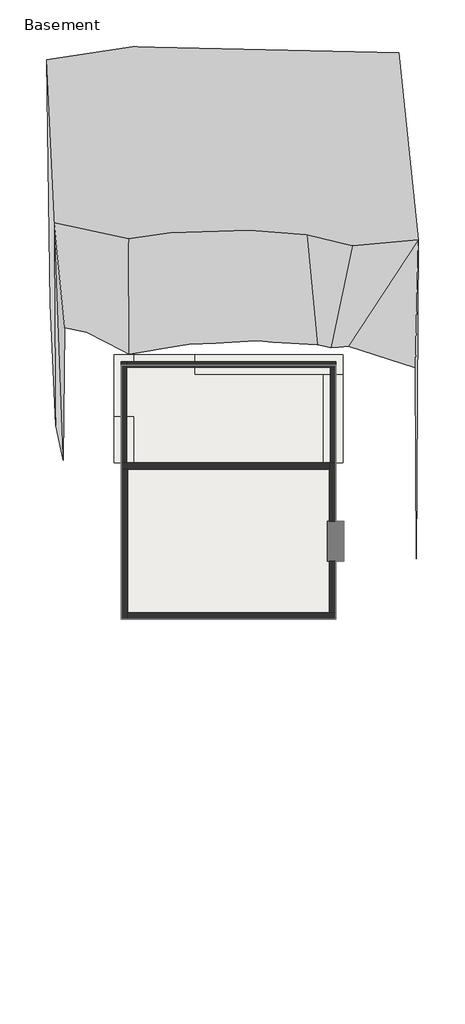
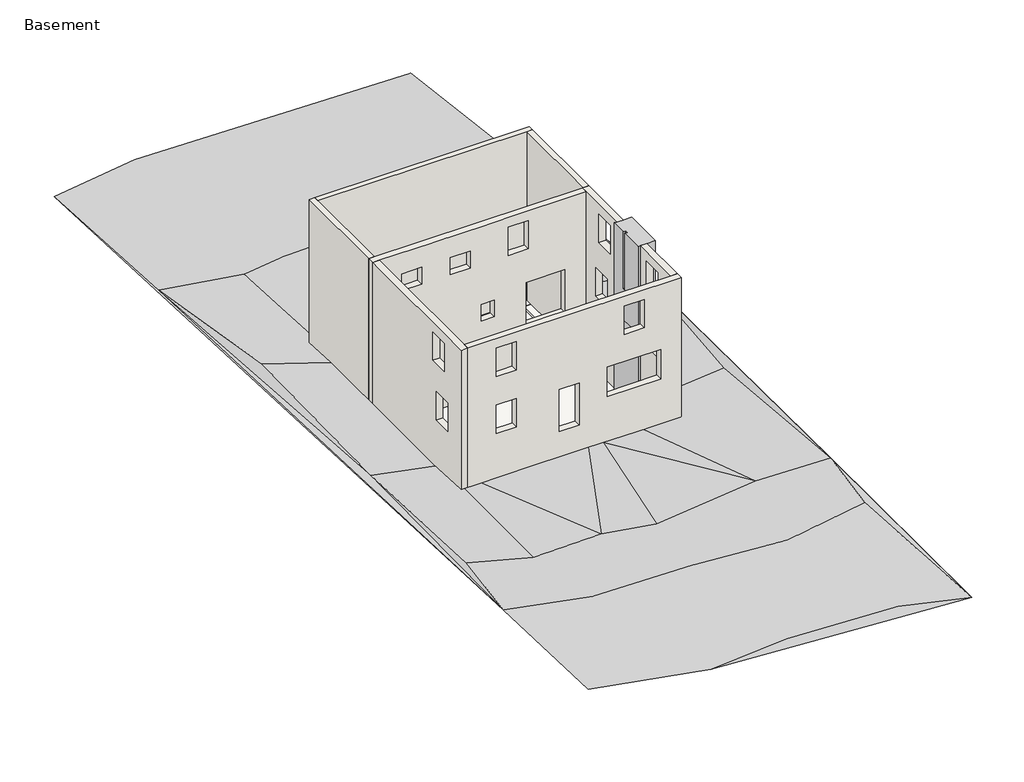
# One storey: 8 walls, 4 proxies, 3 footings, 2 slabs.
"""IFC4 building model written with IfcOpenShell, lengths in millimetres."""

import ifcopenshell
import ifcopenshell.guid

model = None  # the IFC model being written
_history = None  # IfcOwnerHistory: only IFC2X3 demands one
_inside = {}  # id of a spatial element -> (the spatial element, [elements in it])
_under = {}  # id of a project, library or spatial element -> (it, [spatial elements below it])
_declared = {}  # id of a project -> (the project, [libraries it declares])
_typed = {}  # id of a type object -> (the type object, [elements of that type])
_made_of = {}  # id of a material, layer set ... -> (it, [elements and type objects made of it])


def new_model(schema):
    """Start an empty IFC model of exactly this schema.

    Asked for "IFC4X3", IfcOpenShell would pick the latest addendum, in which some entities
    have other attributes; the version numbers below select the first issue.
    IFC2X3 requires an IfcOwnerHistory on every rooted entity: one is made here for all.
    """
    global model, _history
    if schema == "IFC4X3":
        model = ifcopenshell.file(schema_version=(4, 3, 0, 0))
    else:
        model = ifcopenshell.file(schema=schema)
    _inside.clear()
    _under.clear()
    _declared.clear()
    _typed.clear()
    _made_of.clear()
    _history = None
    if model.schema == "IFC2X3":
        org = make("IfcOrganization", Name="unknown")
        user = make(
            "IfcPersonAndOrganization",
            ThePerson=make("IfcPerson", FamilyName="unknown"),
            TheOrganization=org,
        )
        app = make(
            "IfcApplication",
            ApplicationDeveloper=org,
            Version="unknown",
            ApplicationFullName="unknown",
            ApplicationIdentifier="unknown",
        )
        _history = make(
            "IfcOwnerHistory",
            OwningUser=user,
            OwningApplication=app,
            ChangeAction="ADDED",
            CreationDate=0,
        )
    return model


def make(cls, **values):
    """One entity of the class cls with the attributes given. An attribute that is None is left unset."""
    return model.create_entity(
        cls, **{name: value for name, value in values.items() if value is not None}
    )


def rooted(cls, **values):
    """An entity with a GlobalId (a new one), such as an element, a storey or a relation."""
    return make(cls, GlobalId=ifcopenshell.guid.new(), OwnerHistory=_history, **values)


def si_unit(unit_type, name, prefix=None):
    """IfcSIUnit, for example si_unit("LENGTHUNIT", "METRE", prefix="MILLI")."""
    return make("IfcSIUnit", UnitType=unit_type, Prefix=prefix, Name=name)


def assignment(units):
    """IfcUnitAssignment: the units of a project."""
    return None if units is None else make("IfcUnitAssignment", Units=units)


def point(xyz):
    """IfcCartesianPoint."""
    return None if xyz is None else make("IfcCartesianPoint", Coordinates=xyz)


def direction(xyz):
    """IfcDirection."""
    return None if xyz is None else make("IfcDirection", DirectionRatios=xyz)


def frame(location, z_axis=None, x_axis=None):
    """IfcAxis2Placement3D, a coordinate frame: its origin and axes. An axis left out is left unset."""
    return make(
        "IfcAxis2Placement3D",
        Location=point(location),
        Axis=direction(z_axis),
        RefDirection=direction(x_axis),
    )


def origin():
    """The frame at (0, 0, 0) with its axes left unset."""
    return frame((0.0, 0.0, 0.0))


def place(relative_to, where):
    """IfcLocalPlacement: puts the frame where relative to a parent placement (None: the world)."""
    return make(
        "IfcLocalPlacement", PlacementRelTo=relative_to, RelativePlacement=where
    )


def context(
    kind, dimensions, precision=None, world=None, true_north=None, identifier=None
):
    """IfcGeometricRepresentationContext, for example the 3D "Model" context."""
    return make(
        "IfcGeometricRepresentationContext",
        ContextIdentifier=identifier,
        ContextType=kind,
        CoordinateSpaceDimension=dimensions,
        Precision=precision,
        WorldCoordinateSystem=world,
        TrueNorth=true_north,
    )


def project(units=None, contexts=None):
    """IfcProject with its units and contexts."""
    return rooted(
        "IfcProject",
        Name="project",
        RepresentationContexts=contexts,
        UnitsInContext=assignment(units),
    )


def spatial(cls, under=None, at=None, **own):
    """A site, building, storey or space (cls), placed at a placement, below another one or the project."""
    s = rooted(cls, ObjectPlacement=at, **own)
    if under is not None:
        _under.setdefault(under.id(), (under, []))[1].append(s)
    return s


def polyline(points):
    """IfcPolyline through the points."""
    return make("IfcPolyline", Points=[point(p) for p in points])


def point_list(points):
    """IfcCartesianPointList2D or 3D."""
    cls = (
        "IfcCartesianPointList2D" if len(points[0]) == 2 else "IfcCartesianPointList3D"
    )
    return make(cls, CoordList=points)


def outline(outer, holes=None, kind="AREA"):
    """IfcArbitraryClosedProfileDef: a profile drawn as a closed curve; with holes, ...WithVoids."""
    if holes is None:
        return make("IfcArbitraryClosedProfileDef", ProfileType=kind, OuterCurve=outer)
    return make(
        "IfcArbitraryProfileDefWithVoids",
        ProfileType=kind,
        OuterCurve=outer,
        InnerCurves=holes,
    )


def extrude(swept, where, along, depth):
    """IfcExtrudedAreaSolid: the profile swept, set in the frame where, extruded along a direction by depth."""
    return make(
        "IfcExtrudedAreaSolid",
        SweptArea=swept,
        Position=where,
        ExtrudedDirection=direction(along),
        Depth=depth,
    )


def faces_of(points, faces, orient=None, outer=None):
    """IfcFace entities. A face is a list of loops; a loop is a list of indices into points, from 0.

    orient and outer hold one flag for each loop. By default every Orientation is true, the
    first loop of a face is its IfcFaceOuterBound and the others are IfcFaceBound.
    """
    made = []
    for i, loops in enumerate(faces):
        bounds = []
        for j, loop in enumerate(loops):
            is_outer = j == 0 if outer is None else outer[i][j]
            bounds.append(
                make(
                    "IfcFaceOuterBound" if is_outer else "IfcFaceBound",
                    Bound=make("IfcPolyLoop", Polygon=[points[k] for k in loop]),
                    Orientation=True if orient is None else orient[i][j],
                )
            )
        made.append(make("IfcFace", Bounds=bounds))
    return made


def faceted_brep(points, faces, orient=None, outer=None, voids=None):
    """IfcFacetedBrep: a solid bounded by flat faces; with voids (closed shells), ...WithVoids."""
    shared = [point(p) for p in points]
    hull = make("IfcClosedShell", CfsFaces=faces_of(shared, faces, orient, outer))
    if voids is None:
        return make("IfcFacetedBrep", Outer=hull)
    return make(
        "IfcFacetedBrepWithVoids",
        Outer=hull,
        Voids=[
            make(cls, CfsFaces=faces_of(shared, fs, o, b)) for cls, fs, o, b in voids
        ],
    )


def triangles(points, corners, closed=None, point_numbers=None):
    """IfcTriangulatedFaceSet: each triangle names its three corners, points numbered from 1."""
    return make(
        "IfcTriangulatedFaceSet",
        Coordinates=point_list(points),
        Closed=closed,
        CoordIndex=corners,
        PnIndex=point_numbers,
    )


def shape(context_of_items, identifier, shape_type, items):
    """IfcShapeRepresentation: the items that make up one representation, for example the "Body"."""
    return make(
        "IfcShapeRepresentation",
        ContextOfItems=context_of_items,
        RepresentationIdentifier=identifier,
        RepresentationType=shape_type,
        Items=items,
    )


def source(mapping_origin, context_of_items, identifier, shape_type, items):
    """IfcRepresentationMap: a shape defined once, which mapped items show again and again."""
    return make(
        "IfcRepresentationMap",
        MappingOrigin=mapping_origin,
        MappedRepresentation=shape(context_of_items, identifier, shape_type, items),
    )


def transform(
    local_origin,
    x_axis=None,
    y_axis=None,
    z_axis=None,
    scale=None,
    scale2=None,
    scale3=None,
    uniform=True,
):
    """IfcCartesianTransformationOperator3D, or its non-uniform kind. x_axis, y_axis, z_axis: its Axis1, 2, 3."""
    if uniform:
        return make(
            "IfcCartesianTransformationOperator3D",
            Axis1=direction(x_axis),
            Axis2=direction(y_axis),
            LocalOrigin=point(local_origin),
            Scale=scale,
            Axis3=direction(z_axis),
        )
    return make(
        "IfcCartesianTransformationOperator3DnonUniform",
        Axis1=direction(x_axis),
        Axis2=direction(y_axis),
        LocalOrigin=point(local_origin),
        Scale=scale,
        Axis3=direction(z_axis),
        Scale2=scale2,
        Scale3=scale3,
    )


def mapped(mapping_source, mapping_target):
    """IfcMappedItem: shows the shape of a source again, moved by a transform."""
    return make(
        "IfcMappedItem", MappingSource=mapping_source, MappingTarget=mapping_target
    )


def made_of(thing, what):
    """Note that an element or type object is made of a material, layer set ...; save() writes the relation."""
    if what is not None:
        _made_of.setdefault(what.id(), (what, []))[1].append(thing)
    return thing


def element(
    cls,
    number,
    at=None,
    inside=None,
    cuts=None,
    type_object=None,
    material=None,
    context=None,
    identifier="Body",
    shape_type=None,
    held_by="IfcProductDefinitionShape",
    body=None,
    shapes=None,
    **own,
):
    """One element of the class cls, such as IfcWall. Its Tag is "e" and its number.

    at: its placement. inside: the storey or other place that contains it. cuts: it is an
    opening in that element (IfcRelVoidsElement). A single representation is given by context,
    identifier, shape_type and body (its items); several are given by shapes. held_by: the class
    of the entity that holds the representations. save() writes the other relations.
    """
    e = rooted(cls, Tag="e%d" % number, ObjectPlacement=at, **own)
    if body is not None:
        shapes = [shape(context, identifier, shape_type, body)]
    if shapes is not None:
        e.Representation = make(held_by, Representations=shapes)
    if inside is not None:
        _inside.setdefault(inside.id(), (inside, []))[1].append(e)
    if cuts is not None:
        rooted(
            "IfcRelVoidsElement", RelatingBuildingElement=cuts, RelatedOpeningElement=e
        )
    if type_object is not None:
        _typed.setdefault(type_object.id(), (type_object, []))[1].append(e)
    return made_of(e, material)


def aggregate(whole, parts):
    """IfcRelAggregates: a whole, such as a stair, and the parts it consists of."""
    return rooted("IfcRelAggregates", RelatingObject=whole, RelatedObjects=parts)


def save(model, path):
    """Write the relations noted so far, then the file.

    IfcRelAggregates (storeys below a building ...), IfcRelContainedInSpatialStructure (elements
    in a storey), IfcRelDefinesByType, IfcRelAssociatesMaterial and IfcRelDeclares: one each for
    every whole, place, type object, material and project.
    """
    for whole, parts in _under.values():
        aggregate(whole, parts)
    for where, things in _inside.values():
        rooted(
            "IfcRelContainedInSpatialStructure",
            RelatedElements=things,
            RelatingStructure=where,
        )
    for kind, things in _typed.values():
        rooted("IfcRelDefinesByType", RelatedObjects=things, RelatingType=kind)
    for what, things in _made_of.values():
        rooted("IfcRelAssociatesMaterial", RelatedObjects=things, RelatingMaterial=what)
    for by, libraries in _declared.values():
        rooted("IfcRelDeclares", RelatingContext=by, RelatedDefinitions=libraries)
    model.write(path)


def existing_fireplace_existing_fireplace_063a625f(model_context):
    return source(origin(), model_context, "Body", "Brep", [
        faceted_brep([(4450.2196932, 434.2888758, 5486.4), (4069.2196932, 434.2888758, 5486.4), (3764.4196932, 434.2888758, 5486.4), (3662.8196932, 434.2888758, 5486.4), (3662.8196932, -276.9111242, 5486.4), (3767.2567114, -276.9111242, 5486.4), (3767.2567114, -403.9111242, 5486.4), (3662.8196932, -403.9111242, 5486.4), (3662.8196932, -1445.3111242, 5486.4), (3764.4196932, -1445.3111242, 5486.4), (4069.2196932, -1445.3111242, 5486.4), (4450.2196932, -1445.3111242, 5486.4), (4450.2196932, 434.2888758, -2667.0), (4450.2196932, -1445.3111242, -2667.0), (4069.2196932, -1445.3111242, -2667.0), (3764.4196932, -1445.3111242, -2667.0), (3662.8196932, -1445.3111242, -2667.0), (3662.8196932, 434.2888758, -2667.0), (3764.4196932, 434.2888758, -2667.0), (4069.2196932, 434.2888758, -2667.0), (3662.8196932, -403.9111242, 2743.2), (3662.8196932, -276.9111242, 2743.2), (3662.8196932, 154.8888758, 0.0), (3662.8196932, 154.8888758, 1219.2), (3662.8196932, -1165.9111242, 1219.2), (3662.8196932, -1165.9111242, 0.0), (4145.4196932, -20.7631592, 1219.2), (4145.4196932, -990.2590891, 1219.2), (4145.4196932, -990.2590891, 0.0), (4145.4196932, -20.7631592, 0.0), (3767.2567114, -403.9111242, 2743.2), (3767.2567114, -276.9111242, 2743.2)], [[[0, 1, 2, 3, 4, 5, 6, 7, 8, 9, 10, 11]], [[12, 13, 14, 15, 16, 17, 18, 19]], [[3, 2, 1, 0, 12, 19, 18, 17]], [[3, 17, 16, 8, 7, 20, 21, 4], [22, 23, 24, 25]], [[11, 10, 9, 8, 16, 15, 14, 13]], [[0, 11, 13, 12]], [[24, 23, 26, 27]], [[25, 24, 27, 28]], [[27, 26, 29, 28]], [[23, 22, 29, 26]], [[22, 25, 28, 29]], [[6, 30, 20, 7]], [[31, 5, 4, 21]], [[30, 31, 21, 20]], [[30, 6, 5, 31]]]),
    ])


model = new_model("IFC4")

# Units and contexts
model_context = context("Model", 3, world=origin())
ifc_project = project(units=[si_unit("LENGTHUNIT", "METRE", prefix="MILLI")], contexts=[model_context])

# Site, building, storey
site = spatial("IfcSite", under=ifc_project)
building = spatial("IfcBuilding", under=site)
storey = spatial("IfcBuildingStorey", under=building, Name="Basement", Elevation=-2667.0)

# Proxies
placement = place(None, origin())
element("IfcBuildingElementProxy", 1, Name="Building Element Proxy", at=placement, inside=storey, context=model_context, shape_type="Tessellation", body=[
    triangles([(-9474.14729, 22003.2871765, -1727.1999516), (-8916.1412338, -12566.1132111, -939.7999758), (-8632.7724838, -18803.3999359, -1092.1999758), (-3754.3850807, -20036.8885986, -1092.1999758), (7677.2023224, -20906.8378235, -1092.1999758), (7936.7585724, 13587.9496765, -1752.6), (7012.0400162, 22339.8364014, -1727.1999516), (-5437.1349838, 22620.8239014, -1727.1999516), (4069.2196426, 434.2888621, -1346.1999516), (4450.2196426, 434.2888621, -1346.1999516), (4450.2196426, -349.5066825, -1346.1999516), (4450.2196426, -1445.3110531, -1346.1999516), (4069.2196426, -1445.3110531, -1346.1999516), (4069.2196426, -2313.9084709, -1346.1999516), (4069.2196426, -4163.1110046, -1246.6980309), (3428.5651428, -4163.1110046, -1250.4688763), (2349.5500454, -4163.1110046, -1257.7835461), (502.5996998, -4163.1110046, -1235.211668), (-175.7374563, -4163.1110046, -1228.3558365), (-2922.786422, -4163.1110046, -1226.4072636), (-5055.1879486, -4163.1110046, -1242.8984081), (-5852.784613, -4163.1110046, -1243.6517052), (-5989.1803574, -4163.1110046, -1240.8027512), (-5989.1803574, -2711.9263275, -1314.8636375), (-5989.1803574, -2124.4043404, -1346.1999516), (-5989.1803574, 3152.0889954, -1346.1999516), (-5989.1803574, 4989.0600082, -1346.1999516), (-5989.1803574, 6156.3282944, -1346.1999516), (-5989.1803574, 7724.0889954, -1429.2445919), (-5611.7969971, 7724.0889954, -1439.6358181), (-2815.8938187, 7724.0889954, -1415.0254017), (-2474.4123367, 7724.0889954, -1412.4145145), (-1876.9665367, 7724.0889954, -1411.4359406), (391.3462071, 7724.0889954, -1403.6252254), (781.867392, 7724.0889954, -1405.4288944), (3306.7437996, 7724.0889954, -1413.4377079), (3676.8014442, 7724.0889954, -1418.4369667), (4069.2196426, 7724.0889954, -1416.2554138), (4069.2196426, 7529.9159637, -1404.4058464), (4069.2196426, 6299.0253983, -1346.1999516), (4069.2196426, 3152.0889954, -1346.1999516), (-9109.81604, 14372.1750641, -1752.6), (-8549.4287338, -9013.2876297, -939.7999758), (-8523.2349838, -1401.2252266, -1346.1999516), (-8408.9349838, 7414.1625641, -1346.1999516), (-6082.4537338, -10022.9382111, -939.7999758), (-5633.19104, 13643.5125641, -1752.6), (-5382.3662338, -13518.6132111, -939.7999758), (-3671.0413307, 13924.5000641, -1752.6), (-2942.3788307, -9965.7882111, -939.7999758), (-1568.3975807, 21947.7254517, -1727.1999516), (-840.5287823, -13629.7378235, -939.7999758), (-699.241258, -10470.6132111, -939.7999758), (-109.4850414, -19700.3370483, -1092.1999758), (29.4212079, 14035.6246765, -1752.6), (2721.8210724, 13811.7871765, -1752.6), (2805.1648224, 21892.1614014, -1727.1999516), (3252.0462662, -14021.8499359, -939.7999758), (4179.1460724, -9854.6624359, -939.7999758), (4845.1025162, -19962.2745483, -1092.1999758), (4852.2462662, 13306.9621765, -1752.6), (7177.93396, -13294.7757111, -939.7999758), (7289.85271, -1961.6126781, -1346.1999516), (7543.0587662, -9965.7882111, -939.7999758), (7740.7025162, 5059.8998703, -1346.1999516)], [[46, 2, 48], [43, 46, 23], [46, 43, 2], [2, 3, 48], [2, 43, 44], [43, 23, 44], [23, 46, 22], [44, 23, 24], [46, 21, 22], [44, 24, 25], [48, 4, 52], [4, 48, 3], [48, 52, 50], [19, 53, 18], [4, 54, 52], [50, 52, 53], [21, 50, 20], [21, 46, 50], [19, 20, 50], [50, 53, 19], [53, 52, 58], [50, 46, 48], [45, 27, 28], [26, 27, 45], [44, 26, 45], [25, 26, 44], [8, 1, 42], [1, 2, 42], [42, 45, 47], [29, 45, 28], [42, 44, 45], [29, 47, 45], [42, 2, 44], [47, 30, 31], [31, 32, 49], [33, 49, 32], [47, 8, 42], [8, 47, 49], [49, 51, 8], [55, 51, 49], [47, 31, 49], [8, 51, 57], [55, 49, 33], [30, 47, 29], [58, 59, 53], [58, 54, 60], [59, 15, 16], [59, 18, 53], [16, 17, 59], [59, 17, 18], [12, 13, 14], [14, 15, 63], [58, 62, 59], [62, 60, 5], [64, 5, 65], [5, 64, 62], [60, 54, 5], [59, 62, 64], [59, 64, 15], [12, 63, 11], [12, 14, 63], [64, 63, 15], [11, 63, 10], [64, 65, 63], [62, 58, 60], [54, 4, 5], [55, 34, 35], [56, 35, 36], [55, 56, 57], [55, 35, 56], [37, 61, 36], [56, 61, 57], [56, 36, 61], [55, 57, 51], [55, 33, 34], [40, 41, 65], [10, 65, 41], [65, 10, 63], [41, 9, 10], [40, 65, 39], [39, 65, 38], [61, 6, 7], [6, 61, 38], [61, 7, 57], [65, 6, 38], [38, 61, 37], [65, 5, 6], [57, 7, 8], [52, 54, 58]], closed=False),
])
element("IfcBuildingElementProxy", 2, Name="Building Element Proxy", at=placement, inside=storey, context=model_context, shape_type="Tessellation", body=[
    triangles([(4069.2196426, 3152.0889954, -3073.5594864), (4069.2196426, 3152.0889954, -1346.1999516), (4069.2196426, 434.2888621, -3073.5594864), (4069.2196426, 434.2888621, -1346.1999516), (4450.2196426, 434.2888621, -3073.5594864), (4450.2196426, 434.2888621, -1346.1999516), (4450.2196426, -349.5066825, -3073.5594864), (4450.2196426, -349.5066825, -1346.1999516), (4450.2196426, -1445.3110531, -3073.5594864), (4450.2196426, -1445.3110531, -1346.1999516), (4069.2196426, -1445.3110531, -3073.5594864), (4069.2196426, -1445.3110531, -1346.1999516), (4069.2196426, -2313.9084709, -3073.5594864), (4069.2196426, -2313.9084709, -1346.1999516), (4069.2196426, -4163.1110046, -3073.5594864), (4069.2196426, -4163.1110046, -1246.6980309), (3428.5651428, -4163.1110046, -3073.5594864), (3428.5651428, -4163.1110046, -1250.4688763), (2349.5500454, -4163.1110046, -3073.5594864), (2349.5500454, -4163.1110046, -1257.7835461), (502.5996998, -4163.1110046, -3073.5594864), (502.5996998, -4163.1110046, -1235.211668), (-175.7374563, -4163.1110046, -3073.5594864), (-175.7374563, -4163.1110046, -1228.3558365), (-2922.786422, -4163.1110046, -3073.5594864), (-2922.786422, -4163.1110046, -1226.4072636), (-5055.1879486, -4163.1110046, -3073.5594864), (-5055.1879486, -4163.1110046, -1242.8984081), (-5852.784613, -4163.1110046, -3073.5594864), (-5852.784613, -4163.1110046, -1243.6517052), (-5989.1803574, -4163.1110046, -3073.5594864), (-5989.1803574, -4163.1110046, -1240.8027512), (-5989.1803574, -2711.9263275, -3073.5594864), (-5989.1803574, -2711.9263275, -1314.8636375), (-5989.1803574, -2124.4043404, -3073.5594864), (-5989.1803574, -2124.4043404, -1346.1999516), (-5989.1803574, 3152.0889954, -3073.5594864), (-5989.1803574, 3152.0889954, -1346.1999516)], [[1, 4, 2], [1, 3, 4], [3, 6, 4], [3, 5, 6], [5, 8, 6], [5, 7, 8], [7, 10, 8], [7, 9, 10], [9, 12, 10], [9, 11, 12], [11, 14, 12], [11, 13, 14], [13, 16, 14], [13, 15, 16], [15, 18, 16], [15, 17, 18], [17, 20, 18], [17, 19, 20], [19, 22, 20], [19, 21, 22], [21, 24, 22], [21, 23, 24], [23, 26, 24], [23, 25, 26], [25, 28, 26], [25, 27, 28], [27, 30, 28], [27, 29, 30], [29, 32, 30], [29, 31, 32], [31, 34, 32], [31, 33, 34], [33, 36, 34], [33, 35, 36], [35, 38, 36], [35, 37, 38]], closed=False),
    triangles([(4069.2196426, 434.2888621, -3073.5594864), (4069.2196426, 3152.0889954, -3073.5594864), (-5989.1803574, 3152.0889954, -3073.5594864), (-5989.1803574, -4163.1110046, -3073.5594864), (4069.2196426, -4163.1110046, -3073.5594864), (4069.2196426, -1445.3110531, -3073.5594864), (4450.2196426, -1445.3110531, -3073.5594864), (4450.2196426, 434.2888621, -3073.5594864)], [[4, 6, 3], [6, 4, 5], [3, 1, 2], [1, 3, 6], [6, 7, 1], [8, 1, 7]], closed=False),
])
element("IfcBuildingElementProxy", 3, Name="Building Element Proxy", at=placement, inside=storey, context=model_context, shape_type="Tessellation", body=[
    triangles([(-5989.1803574, 3152.0889954, -3073.5594864), (-5989.1803574, 3152.0889954, -1346.1999516), (-5989.1803574, 4989.0600082, -3073.5594864), (-5989.1803574, 4989.0600082, -1346.1999516), (-5989.1803574, 6156.3282944, -3073.5594864), (-5989.1803574, 6156.3282944, -1346.1999516), (-5989.1803574, 7724.0889954, -3073.5594864), (-5989.1803574, 7724.0889954, -1429.2445919), (-5611.7969971, 7724.0889954, -3073.5594864), (-5611.7969971, 7724.0889954, -1439.6358181), (-2815.8938187, 7724.0889954, -3073.5594864), (-2815.8938187, 7724.0889954, -1415.0254017), (-2474.4123367, 7724.0889954, -3073.5594864), (-2474.4123367, 7724.0889954, -1412.4145145), (-1876.9665367, 7724.0889954, -3073.5594864), (-1876.9665367, 7724.0889954, -1411.4359406), (391.3462071, 7724.0889954, -3073.5594864), (391.3462071, 7724.0889954, -1403.6252254), (781.867392, 7724.0889954, -3073.5594864), (781.867392, 7724.0889954, -1405.4288944), (3306.7437996, 7724.0889954, -3073.5594864), (3306.7437996, 7724.0889954, -1413.4377079), (3676.8014442, 7724.0889954, -3073.5594864), (3676.8014442, 7724.0889954, -1418.4369667), (4069.2196426, 7724.0889954, -3073.5594864), (4069.2196426, 7724.0889954, -1416.2554138), (4069.2196426, 7529.9159637, -3073.5594864), (4069.2196426, 7529.9159637, -1404.4058464), (4069.2196426, 6299.0253983, -3073.5594864), (4069.2196426, 6299.0253983, -1346.1999516), (4069.2196426, 3152.0889954, -3073.5594864), (4069.2196426, 3152.0889954, -1346.1999516)], [[1, 4, 2], [1, 3, 4], [3, 6, 4], [3, 5, 6], [5, 8, 6], [5, 7, 8], [7, 10, 8], [7, 9, 10], [9, 12, 10], [9, 11, 12], [11, 14, 12], [11, 13, 14], [13, 16, 14], [13, 15, 16], [15, 18, 16], [15, 17, 18], [17, 20, 18], [17, 19, 20], [19, 22, 20], [19, 21, 22], [21, 24, 22], [21, 23, 24], [23, 26, 24], [23, 25, 26], [25, 28, 26], [25, 27, 28], [27, 30, 28], [27, 29, 30], [29, 32, 30], [29, 31, 32]], closed=False),
    triangles([(-5989.1803574, 7724.0889954, -3073.5594864), (-5989.1803574, 3152.0889954, -3073.5594864), (4069.2196426, 3152.0889954, -3073.5594864), (4069.2196426, 7724.0889954, -3073.5594864)], [[1, 2, 4], [3, 4, 2]], closed=False),
])
existing_fireplace_existing_fireplace_shape = existing_fireplace_existing_fireplace_063a625f(model_context)
element("IfcBuildingElementProxy", 4, Name="Existing Fireplace : Existing Fireplace", ObjectType="Existing Fireplace : Existing Fireplace", at=placement, inside=storey, context=model_context, shape_type="MappedRepresentation", body=[
    mapped(existing_fireplace_existing_fireplace_shape, transform((0.0, 0.0, 0.0), x_axis=(1.0, 0.0, 0.0), y_axis=(0.0, 1.0, 0.0), z_axis=(0.0, 0.0, 1.0))),
])

# Footings
element("IfcFooting", 5, ObjectType="Bearing Footing - 36\" x 12\"", at=placement, inside=storey, context=model_context, shape_type="Brep", body=[
    faceted_brep([(-5404.9803068, 3152.0888758, -2667.0), (-6319.3803068, 3152.0888758, -2667.0), (-6319.3803068, 3152.0888758, -2971.8), (-5404.9803068, 3152.0888758, -2971.8), (-6319.3803068, 5311.0888758, -2667.0), (-5404.9803068, 5311.0888758, -2667.0), (-5404.9803068, 5311.0888758, -2971.8), (-6319.3803068, 5311.0888758, -2971.8)], [[[0, 1, 2, 3]], [[4, 5, 6, 7]], [[0, 5, 4, 1]], [[2, 1, 4, 7]], [[3, 2, 7, 6]], [[0, 3, 6, 5]]]),
    faceted_brep([(-5404.9803068, 5311.0888758, -3124.2), (-6319.3803068, 5311.0888758, -3124.2), (-6319.3803068, 5311.0888758, -3429.0), (-5404.9803068, 5311.0888758, -3429.0), (-5404.9803068, 7292.2888758, -3124.2), (-5404.9803068, 8206.6888758, -3124.2), (-6319.3803068, 8206.6888758, -3124.2), (-6319.3803068, 8206.6888758, -3429.0), (-5404.9803068, 8206.6888758, -3429.0), (-5404.9803068, 7292.2888758, -3429.0)], [[[0, 1, 2, 3]], [[0, 4, 5, 6, 1]], [[2, 1, 6, 7]], [[3, 2, 7, 8, 9]], [[0, 3, 9, 8, 5, 4]], [[6, 5, 8, 7]]]),
])
element("IfcFooting", 6, ObjectType="Bearing Footing - 36\" x 12\"", at=placement, inside=storey, context=model_context, shape_type="Brep", body=[
    faceted_brep([(-2509.3803068, 8206.6888758, -3429.0), (-2509.3803068, 8206.6888758, -3124.2), (-2509.3803068, 7292.2888758, -3124.2), (-2509.3803068, 7292.2888758, -3429.0), (-5404.9803068, 8206.6888758, -3124.2), (-5404.9803068, 7292.2888758, -3124.2), (-5404.9803068, 8206.6888758, -3429.0), (-5404.9803068, 7292.2888758, -3429.0)], [[[0, 1, 2, 3]], [[2, 1, 4, 5]], [[1, 0, 6, 4]], [[0, 3, 7, 6]], [[3, 2, 5, 7]], [[5, 4, 6, 7]]]),
    faceted_brep([(-2509.3803068, 8206.6888758, -2667.0), (-2509.3803068, 8206.6888758, -2971.8), (-2509.3803068, 7292.2888758, -2971.8), (-2509.3803068, 7292.2888758, -2667.0), (4399.4196932, 8206.6888758, -2667.0), (3485.0196932, 7292.2888758, -2667.0), (4399.4196932, 7292.2888758, -2667.0), (4399.4196932, 8206.6888758, -2971.8), (4399.4196932, 7292.2888758, -2971.8), (3485.0196932, 7292.2888758, -2971.8)], [[[0, 1, 2, 3]], [[4, 0, 3, 5, 6]], [[1, 0, 4, 7]], [[2, 1, 7, 8, 9]], [[3, 2, 9, 8, 6, 5]], [[4, 6, 8, 7]]]),
])
element("IfcFooting", 7, ObjectType="Bearing Footing - 36\" x 12\"", at=placement, inside=storey, context=model_context, shape_type="SweptSolid", body=[
    extrude(outline(polyline([(4399.4196932, 3152.0888758), (3485.0196932, 3152.0888758), (3485.0196932, 7292.2888758), (4399.4196932, 7292.2888758), (4399.4196932, 3152.0888758)])), frame((0.0, 0.0, -2971.8), z_axis=(0.0, 0.0, 1.0), x_axis=(1.0, 0.0, 0.0)), (0.0, 0.0, 1.0), 304.8),
])

# Slabs
element("IfcSlab", 8, ObjectType="Pad 1", at=placement, inside=storey, context=model_context, shape_type="SweptSolid", body=[
    extrude(outline(polyline([(4069.2196932, 434.2888758), (4450.2196932, 434.2888758), (4450.2196932, -1445.3111242), (4069.2196932, -1445.3111242), (4069.2196932, -4163.1111242), (-5989.1803068, -4163.1111242), (-5989.1803068, 3152.0888758), (4069.2196932, 3152.0888758), (4069.2196932, 434.2888758)])), frame((0.0, 0.0, -3073.4), z_axis=(0.0, 0.0, 1.0), x_axis=(1.0, 0.0, 0.0)), (0.0, 0.0, 1.0), 304.8),
])
element("IfcSlab", 9, ObjectType="Pad 1", at=placement, inside=storey, context=model_context, shape_type="SweptSolid", body=[
    extrude(outline(polyline([(-5989.1803068, 7724.0888758), (4069.2196932, 7724.0888758), (4069.2196932, 3152.0888758), (-5989.1803068, 3152.0888758), (-5989.1803068, 7724.0888758)])), frame((0.0, 0.0, -3073.4), z_axis=(0.0, 0.0, 1.0), x_axis=(1.0, 0.0, 0.0)), (0.0, 0.0, 1.0), 304.8),
])

# Walls
element("IfcWall", 10, ObjectType="Generic - 10\"", at=placement, inside=storey, context=model_context, shape_type="Brep", body=[
    faceted_brep([(-5735.1803068, 3152.0888758, -2667.0), (-5735.1803068, 5311.0888758, -2667.0), (-5735.1803068, 5311.0888758, -3124.2), (-5735.1803068, 7622.4888758, -3124.2), (-5735.1803068, 7876.4888758, -3124.2), (-5735.1803068, 7876.4888758, 5486.4), (-5735.1803068, 7622.4888758, 5486.4), (-5735.1803068, 3152.0888758, 5486.4), (-5989.1803068, 3152.0888758, -2667.0), (-5989.1803068, 3152.0888758, 5486.4), (-5989.1803068, 7876.4888758, 5486.4), (-5989.1803068, 7876.4888758, -3124.2), (-5989.1803068, 5311.0888758, -3124.2), (-5989.1803068, 5311.0888758, -2667.0)], [[[0, 1, 2, 3, 4, 5, 6, 7]], [[8, 9, 10, 11, 12, 13]], [[1, 0, 8, 13]], [[2, 1, 13, 12]], [[4, 3, 2, 12, 11]], [[7, 6, 5, 10, 9]], [[5, 4, 11, 10]], [[0, 7, 9, 8]]]),
])
element("IfcWall", 11, ObjectType="Generic - 10\"", at=placement, inside=storey, context=model_context, shape_type="Brep", body=[
    faceted_brep([(-5735.1803068, 7622.4888758, -3124.2), (-2509.3803068, 7622.4888758, -3124.2), (-2509.3803068, 7622.4888758, -2667.0), (3815.2196932, 7622.4888758, -2667.0), (4069.2196932, 7622.4888758, -2667.0), (4069.2196932, 7622.4888758, 5486.4), (3815.2196932, 7622.4888758, 5486.4), (-5735.1803068, 7622.4888758, 5486.4), (-5735.1803068, 7876.4888758, -3124.2), (-5735.1803068, 7876.4888758, 5486.4), (4069.2196932, 7876.4888758, 5486.4), (4069.2196932, 7876.4888758, -2667.0), (-2509.3803068, 7876.4888758, -2667.0), (-2509.3803068, 7876.4888758, -3124.2)], [[[0, 1, 2, 3, 4, 5, 6, 7]], [[8, 9, 10, 11, 12, 13]], [[1, 0, 8, 13]], [[2, 1, 13, 12]], [[4, 3, 2, 12, 11]], [[7, 6, 5, 10, 9]], [[5, 4, 11, 10]], [[0, 7, 9, 8]]]),
])
element("IfcWall", 12, ObjectType="Generic - 10\"", at=placement, inside=storey, context=model_context, shape_type="SweptSolid", body=[
    extrude(outline(polyline([(3815.2196932, 3152.0888758), (3815.2196932, 7622.4888758), (4069.2196932, 7622.4888758), (4069.2196932, 3152.0888758), (3815.2196932, 3152.0888758)])), frame((0.0, 0.0, -2667.0), z_axis=(0.0, 0.0, 1.0), x_axis=(1.0, 0.0, 0.0)), (0.0, 0.0, 1.0), 8153.4),
])
element("IfcWall", 13, ObjectType="Generic - 12\"", at=placement, inside=storey, context=model_context, shape_type="Brep", body=[
    faceted_brep([(-5989.1803068, 2847.2888758, -2667.0), (-5684.3803068, 2847.2888758, -2667.0), (3764.4196932, 2847.2888758, -2667.0), (3764.4196932, 2847.2888758, 5486.4), (56.0196932, 2847.2888758, 5486.4), (-70.9803068, 2847.2888758, 5486.4), (-680.5803068, 2847.2888758, 5486.4), (-807.5803068, 2847.2888758, 5486.4), (-3169.7803068, 2847.2888758, 5486.4), (-3296.7803068, 2847.2888758, 5486.4), (-5684.3803068, 2847.2888758, 5486.4), (-5989.1803068, 2847.2888758, 5486.4), (1021.2196932, 2847.2888758, 0.0), (1021.2196932, 2847.2888758, 2057.4), (2799.2196932, 2847.2888758, 2057.4), (2799.2196932, 2847.2888758, 0.0), (-4160.3803068, 2847.2888758, 0.0), (-5023.9803068, 2847.2888758, 0.0), (-5023.9803068, 2847.2888758, 2032.0), (-4160.3803068, 2847.2888758, 2032.0), (-1036.1803068, 2847.2888758, 914.4), (-1036.1803068, 2847.2888758, 1727.2), (-426.5803068, 2847.2888758, 1727.2), (-426.5803068, 2847.2888758, 914.4), (-3919.0803068, 2847.2888758, 914.4), (-3919.0803068, 2847.2888758, 1727.2), (-3004.6803068, 2847.2888758, 1727.2), (-3004.6803068, 2847.2888758, 914.4), (208.4196932, 2847.2888758, 3657.6), (208.4196932, 2847.2888758, 5029.2), (1122.8196932, 2847.2888758, 5029.2), (1122.8196932, 2847.2888758, 3657.6), (-2433.1803068, 2847.2888758, 3657.6), (-2433.1803068, 2847.2888758, 4470.4), (-1518.7803068, 2847.2888758, 4470.4), (-1518.7803068, 2847.2888758, 3657.6), (-4668.3803068, 2847.2888758, 3657.6), (-4668.3803068, 2847.2888758, 4470.4), (-3753.9803068, 2847.2888758, 4470.4), (-3753.9803068, 2847.2888758, 3657.6), (3764.4196932, 3152.0888758, -2667.0), (-5989.1803068, 3152.0888758, -2667.0), (-5989.1803068, 3152.0888758, 5486.4), (3764.4196932, 3152.0888758, 5486.4), (1021.2196932, 3152.0888758, 2057.4), (1021.2196932, 3152.0888758, 0.0), (2799.2196932, 3152.0888758, 0.0), (2799.2196932, 3152.0888758, 2057.4), (-5023.9803068, 3152.0888758, 0.0), (-4160.3803068, 3152.0888758, 0.0), (-4160.3803068, 3152.0888758, 2032.0), (-5023.9803068, 3152.0888758, 2032.0), (-1036.1803068, 3152.0888758, 1727.2), (-1036.1803068, 3152.0888758, 914.4), (-426.5803068, 3152.0888758, 914.4), (-426.5803068, 3152.0888758, 1727.2), (-3919.0803068, 3152.0888758, 1727.2), (-3919.0803068, 3152.0888758, 914.4), (-3004.6803068, 3152.0888758, 914.4), (-3004.6803068, 3152.0888758, 1727.2), (208.4196932, 3152.0888758, 5029.2), (208.4196932, 3152.0888758, 3657.6), (1122.8196932, 3152.0888758, 3657.6), (1122.8196932, 3152.0888758, 5029.2), (-2433.1803068, 3152.0888758, 4470.4), (-2433.1803068, 3152.0888758, 3657.6), (-1518.7803068, 3152.0888758, 3657.6), (-1518.7803068, 3152.0888758, 4470.4), (-4668.3803068, 3152.0888758, 4470.4), (-4668.3803068, 3152.0888758, 3657.6), (-3753.9803068, 3152.0888758, 3657.6), (-3753.9803068, 3152.0888758, 4470.4)], [[[0, 1, 2, 3, 4, 5, 6, 7, 8, 9, 10, 11], [12, 13, 14, 15], [16, 17, 18, 19], [20, 21, 22, 23], [24, 25, 26, 27], [28, 29, 30, 31], [32, 33, 34, 35], [36, 37, 38, 39]], [[40, 41, 42, 43], [44, 45, 46, 47], [48, 49, 50, 51], [52, 53, 54, 55], [56, 57, 58, 59], [60, 61, 62, 63], [64, 65, 66, 67], [68, 69, 70, 71]], [[2, 1, 0, 41, 40]], [[11, 10, 9, 8, 7, 6, 5, 4, 3, 43, 42]], [[0, 11, 42, 41]], [[3, 2, 40, 43]], [[44, 13, 12, 45]], [[13, 44, 47, 14]], [[14, 47, 46, 15]], [[45, 12, 15, 46]], [[17, 16, 49, 48]], [[18, 17, 48, 51]], [[19, 18, 51, 50]], [[16, 19, 50, 49]], [[53, 52, 21, 20]], [[54, 53, 20, 23]], [[55, 54, 23, 22]], [[52, 55, 22, 21]], [[57, 56, 25, 24]], [[58, 57, 24, 27]], [[59, 58, 27, 26]], [[56, 59, 26, 25]], [[60, 29, 28, 61]], [[61, 28, 31, 62]], [[62, 31, 30, 63]], [[29, 60, 63, 30]], [[33, 32, 65, 64]], [[32, 35, 66, 65]], [[35, 34, 67, 66]], [[34, 33, 64, 67]], [[37, 36, 69, 68]], [[36, 39, 70, 69]], [[39, 38, 71, 70]], [[38, 37, 68, 71]]]),
])
element("IfcWall", 14, ObjectType="Generic - 12\"", at=placement, inside=storey, context=model_context, shape_type="Brep", body=[
    faceted_brep([(-5684.3803068, -4163.1111242, -2667.0), (-5684.3803068, -3858.3111242, -2667.0), (-5684.3803068, 2847.2888758, -2667.0), (-5684.3803068, 2847.2888758, 5486.4), (-5684.3803068, 1450.2888758, 5486.4), (-5684.3803068, 1323.2888758, 5486.4), (-5684.3803068, -3858.3111242, 5486.4), (-5684.3803068, -4163.1111242, 5486.4), (-5684.3803068, -3096.3111242, 914.4), (-5684.3803068, -3096.3111242, 2286.0), (-5684.3803068, -2181.9111242, 2286.0), (-5684.3803068, -2181.9111242, 914.4), (-5684.3803068, -2842.3111242, 3657.6), (-5684.3803068, -2842.3111242, 5029.2), (-5684.3803068, -1927.9111242, 5029.2), (-5684.3803068, -1927.9111242, 3657.6), (-5989.1803068, 2847.2888758, -2667.0), (-5989.1803068, -4163.1111242, -2667.0), (-5989.1803068, -4163.1111242, 5486.4), (-5989.1803068, 2847.2888758, 5486.4), (-5989.1803068, -3096.3111242, 2286.0), (-5989.1803068, -3096.3111242, 914.4), (-5989.1803068, -2181.9111242, 914.4), (-5989.1803068, -2181.9111242, 2286.0), (-5989.1803068, -2842.3111242, 5029.2), (-5989.1803068, -2842.3111242, 3657.6), (-5989.1803068, -1927.9111242, 3657.6), (-5989.1803068, -1927.9111242, 5029.2)], [[[0, 1, 2, 3, 4, 5, 6, 7], [8, 9, 10, 11], [12, 13, 14, 15]], [[16, 17, 18, 19], [20, 21, 22, 23], [24, 25, 26, 27]], [[2, 1, 0, 17, 16]], [[7, 6, 5, 4, 3, 19, 18]], [[0, 7, 18, 17]], [[3, 2, 16, 19]], [[21, 20, 9, 8]], [[22, 21, 8, 11]], [[23, 22, 11, 10]], [[20, 23, 10, 9]], [[24, 13, 12, 25]], [[25, 12, 15, 26]], [[26, 15, 14, 27]], [[13, 24, 27, 14]]]),
])
element("IfcWall", 15, ObjectType="Generic - 12\"", at=placement, inside=storey, context=model_context, shape_type="Brep", body=[
    faceted_brep([(4069.2196932, -3858.3111242, -2667.0), (3764.4196932, -3858.3111242, -2667.0), (-5684.3803068, -3858.3111242, -2667.0), (-5684.3803068, -3858.3111242, 5486.4), (-2179.1803068, -3858.3111242, 5486.4), (-2052.1803068, -3858.3111242, 5486.4), (-807.5803068, -3858.3111242, 5486.4), (-680.5803068, -3858.3111242, 5486.4), (-70.9803068, -3858.3111242, 5486.4), (56.0196932, -3858.3111242, 5486.4), (3764.4196932, -3858.3111242, 5486.4), (4069.2196932, -3858.3111242, 5486.4), (-1518.7803068, -3858.3111242, 0.0), (-604.3803068, -3858.3111242, 0.0), (-604.3803068, -3858.3111242, 2032.0), (-1518.7803068, -3858.3111242, 2032.0), (-3474.5803068, -3858.3111242, 914.4), (-3474.5803068, -3858.3111242, 2286.0), (-4388.9803068, -3858.3111242, 2286.0), (-4388.9803068, -3858.3111242, 914.4), (691.0196932, -3858.3111242, 2336.8), (691.0196932, -3858.3111242, 914.4), (3129.4196932, -3858.3111242, 914.4), (3129.4196932, -3858.3111242, 2336.8), (2367.4196932, -3858.3111242, 3657.6), (2367.4196932, -3858.3111242, 5029.2), (1453.0196932, -3858.3111242, 5029.2), (1453.0196932, -3858.3111242, 3657.6), (-3474.5803068, -3858.3111242, 3657.6), (-3474.5803068, -3858.3111242, 5029.2), (-4388.9803068, -3858.3111242, 5029.2), (-4388.9803068, -3858.3111242, 3657.6), (-5684.3803068, -4163.1111242, -2667.0), (4069.2196932, -4163.1111242, -2667.0), (4069.2196932, -4163.1111242, 5486.4), (-5684.3803068, -4163.1111242, 5486.4), (-604.3803068, -4163.1111242, 0.0), (-1518.7803068, -4163.1111242, 0.0), (-1518.7803068, -4163.1111242, 2032.0), (-604.3803068, -4163.1111242, 2032.0), (-3474.5803068, -4163.1111242, 2286.0), (-3474.5803068, -4163.1111242, 914.4), (-4388.9803068, -4163.1111242, 914.4), (-4388.9803068, -4163.1111242, 2286.0), (691.0196932, -4163.1111242, 914.4), (691.0196932, -4163.1111242, 2336.8), (3129.4196932, -4163.1111242, 2336.8), (3129.4196932, -4163.1111242, 914.4), (2367.4196932, -4163.1111242, 5029.2), (2367.4196932, -4163.1111242, 3657.6), (1453.0196932, -4163.1111242, 3657.6), (1453.0196932, -4163.1111242, 5029.2), (-3474.5803068, -4163.1111242, 5029.2), (-3474.5803068, -4163.1111242, 3657.6), (-4388.9803068, -4163.1111242, 3657.6), (-4388.9803068, -4163.1111242, 5029.2)], [[[0, 1, 2, 3, 4, 5, 6, 7, 8, 9, 10, 11], [12, 13, 14, 15], [16, 17, 18, 19], [20, 21, 22, 23], [24, 25, 26, 27], [28, 29, 30, 31]], [[32, 33, 34, 35], [36, 37, 38, 39], [40, 41, 42, 43], [44, 45, 46, 47], [48, 49, 50, 51], [52, 53, 54, 55]], [[2, 1, 0, 33, 32]], [[11, 10, 9, 8, 7, 6, 5, 4, 3, 35, 34]], [[0, 11, 34, 33]], [[3, 2, 32, 35]], [[37, 36, 13, 12]], [[38, 37, 12, 15]], [[39, 38, 15, 14]], [[36, 39, 14, 13]], [[41, 40, 17, 16]], [[42, 41, 16, 19]], [[43, 42, 19, 18]], [[40, 43, 18, 17]], [[21, 44, 47, 22]], [[45, 20, 23, 46]], [[20, 45, 44, 21]], [[22, 47, 46, 23]], [[25, 24, 49, 48]], [[24, 27, 50, 49]], [[27, 26, 51, 50]], [[26, 25, 48, 51]], [[52, 29, 28, 53]], [[53, 28, 31, 54]], [[54, 31, 30, 55]], [[29, 52, 55, 30]]]),
])
element("IfcWall", 16, ObjectType="Generic - 12\"", at=placement, inside=storey, context=model_context, shape_type="Brep", body=[
    faceted_brep([(3764.4196932, 3152.0888758, -2667.0), (3764.4196932, 2847.2888758, -2667.0), (3764.4196932, 434.2888758, -2667.0), (3764.4196932, 434.2888758, 5486.4), (3764.4196932, 2847.2888758, 5486.4), (3764.4196932, 3152.0888758, 5486.4), (3764.4196932, 2085.2888758, 914.4), (3764.4196932, 2085.2888758, 2286.0), (3764.4196932, 1170.8888758, 2286.0), (3764.4196932, 1170.8888758, 914.4), (3764.4196932, 1831.2888758, 3657.6), (3764.4196932, 1831.2888758, 5029.2), (3764.4196932, 916.8888758, 5029.2), (3764.4196932, 916.8888758, 3657.6), (4069.2196932, 434.2888758, -2667.0), (4069.2196932, 3152.0888758, -2667.0), (4069.2196932, 3152.0888758, 5486.4), (4069.2196932, 434.2888758, 5486.4), (4069.2196932, 2085.2888758, 2286.0), (4069.2196932, 2085.2888758, 914.4), (4069.2196932, 1170.8888758, 914.4), (4069.2196932, 1170.8888758, 2286.0), (4069.2196932, 1831.2888758, 5029.2), (4069.2196932, 1831.2888758, 3657.6), (4069.2196932, 916.8888758, 3657.6), (4069.2196932, 916.8888758, 5029.2)], [[[0, 1, 2, 3, 4, 5], [6, 7, 8, 9], [10, 11, 12, 13]], [[14, 15, 16, 17], [18, 19, 20, 21], [22, 23, 24, 25]], [[2, 1, 0, 15, 14]], [[3, 2, 14, 17]], [[5, 4, 3, 17, 16]], [[0, 5, 16, 15]], [[19, 18, 7, 6]], [[20, 19, 6, 9]], [[21, 20, 9, 8]], [[18, 21, 8, 7]], [[22, 11, 10, 23]], [[23, 10, 13, 24]], [[24, 13, 12, 25]], [[11, 22, 25, 12]]]),
])
element("IfcWall", 17, ObjectType="Generic - 12\"", at=placement, inside=storey, context=model_context, shape_type="SweptSolid", body=[
    extrude(outline(polyline([(-1445.3111242, -2667.0), (-3858.3111242, -2667.0), (-3858.3111242, 5486.4), (-1445.3111242, 5486.4), (-1445.3111242, -2667.0)]), holes=[polyline([(-2181.9111242, 2286.0), (-3096.3111242, 2286.0), (-3096.3111242, 914.4), (-2181.9111242, 914.4), (-2181.9111242, 2286.0)]), polyline([(-1927.9111242, 3657.6), (-1927.9111242, 5029.2), (-2842.3111242, 5029.2), (-2842.3111242, 3657.6), (-1927.9111242, 3657.6)])]), frame((3764.4196932, 0.0, 0.0), z_axis=(1.0, 0.0, 0.0), x_axis=(0.0, 1.0, 0.0)), (0.0, 0.0, 1.0), 304.8),
])

save(model, "model.ifc")

# Revit data of these elements
# Project information
#   Organization Name = "G3B Press"
#   Organization Description = "Paul F. Aubin Cosulting Services, Inc."
#   Building Name = "Revit Essentials for Architecture"
#   Author = "Paul F. Aubin"
#   Author Website = "https://www.paulaubin.com"
#   Copyright = "Copyright © 2020 Paul F Aubin, all rights reserved"
#   Project Issue Date = "8/1/2020"
#   Project Status = "Design Development"
#   Client Name = "Column Grids and Structural Layout"
#   Project Address = "789 Main ST\nAnytown, IL 60000"
#   Project Name = "06 Residential_Complete"
#   Project Number = "2020.03A"
# Type "Bearing Footing - 36\" x 12\""
#   Assembly Code = "A1010110"
# Type "Pad 1"
#   Layers, outside or top first: 1' - 0" no material (function 1)
# Type "Generic - 10\""
#   Assembly Code = "B2010"
#   Layers, outside or top first: 0' - 10" no material (function 1)
# Type "Generic - 12\""
#   Assembly Code = "B2010"
#   Layers, outside or top first: 1' - 0" no material (function 1)
# Elements 1, 2, 3 (IfcBuildingElementProxy)
#   Material = none
#   Phase Created = New Construction
# Element 4 (IfcBuildingElementProxy, "Existing Fireplace : Existing Fireplace")
#   Phase Created = Existing
# Element 5 (IfcFooting, "Bearing Footing - 36\" x 12\"")
#   Phase Created = New Construction
#   Materials on its faces: "Concrete, Cast-in-Place gray"
# Elements 6, 7 (IfcFooting, "Bearing Footing - 36\" x 12\"")
#   Comments = ""
#   Phase Created = New Construction
#   Materials on its faces: "Concrete, Cast-in-Place gray"
# Elements 8, 9 (IfcSlab, "Pad 1")
#   built-in parameter 1012502 = -0.333333 (stored number, unit not read)
#   Phase Created = New Construction
# Elements 10, 11, 12 (IfcWall, "Generic - 10\"")
#   Top Offset = 0' - 0"
#   Base Offset = 0' - 0"
#   wall height = 26' - 9"
#   Phase Created = New Construction
#   Base Constraint = Basement
#   Top Constraint = Roof
#   Materials on its faces: "Default Wall"
# Elements 13, 14, 15, 16, 17 (IfcWall, "Generic - 12\"")
#   Top Offset = 0' - 0"
#   Base Offset = 0' - 0"
#   wall height = 26' - 9"
#   Phase Created = Existing
#   Base Constraint = Basement
#   Top Constraint = Roof
#   Materials on its faces: "Default Wall"
# Materials
#   "Concrete, Cast-in-Place gray": class "Concrete", colour RGB 192 192 192, transparency 0, Description = "Cast-in-place concrete", Cost = 0
#   "Default Wall": class "Miscellaneous", colour RGB 128 128 128, transparency 0, Cost = 0
